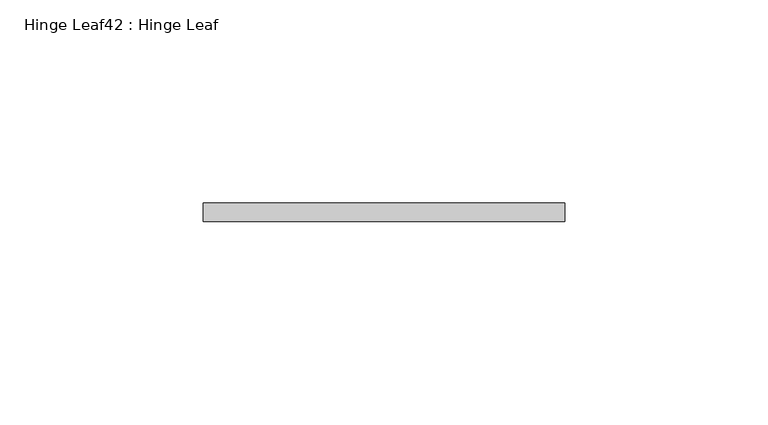
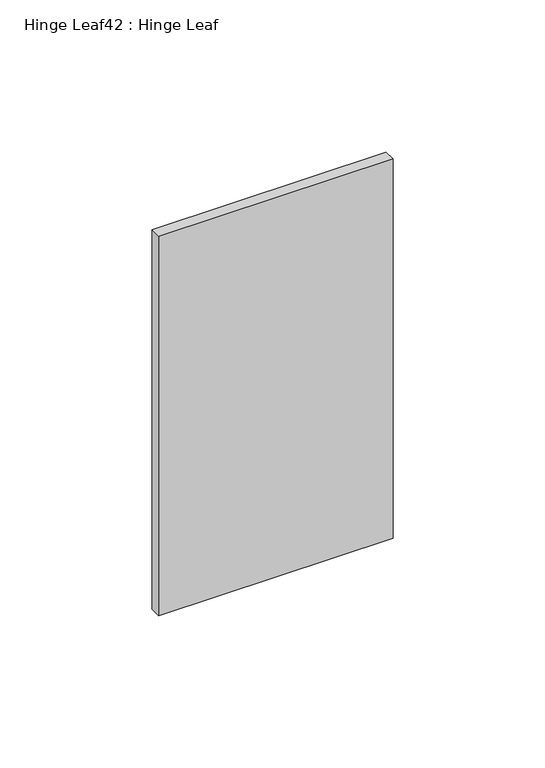
"""IFC4 building model written with IfcOpenShell, lengths in millimetres: proxy geometry, Hinge Leaf42 : Hinge Leaf."""

from ifc_helpers import new_model, si_unit, frame, origin, place, context, project, spatial, polyline, outline, extrude, source, transform, mapped, element, save


def hinge_leaf42_hinge_leaf_9b6187f5(model_context):
    return source(origin(), model_context, "Body", "SweptSolid", [
        extrude(outline(polyline([(587327.7934739, -534104.7943841), (587416.6934739, -534104.7943841), (587416.6934739, -534109.3663841), (587327.7934739, -534109.3663841), (587327.7934739, -534104.7943841)])), frame((0.0, 0.0, 1123.95), z_axis=(0.0, 0.0, 1.0), x_axis=(1.0, 0.0, 0.0)), (0.0, 0.0, 1.0), 152.4),
    ])


if __name__ == "__main__":
    model = new_model("IFC4")
    model_context = context("Model", 3, world=origin())
    ifc_project = project(units=[si_unit("LENGTHUNIT", "METRE", prefix="MILLI")], contexts=[model_context])
    site = spatial("IfcSite", under=ifc_project)
    building = spatial("IfcBuilding", under=site)
    placement = place(None, origin())
    hinge_leaf42_hinge_leaf_shape = hinge_leaf42_hinge_leaf_9b6187f5(model_context)
    element("IfcBuildingElementProxy", 1, Name="Hinge Leaf42 : Hinge Leaf", ObjectType="Hinge Leaf42 : Hinge Leaf", at=placement, inside=building, context=model_context, shape_type="MappedRepresentation", body=[
        mapped(hinge_leaf42_hinge_leaf_shape, transform((0.0, 0.0, 0.0), x_axis=(1.0, 0.0, 0.0), y_axis=(0.0, 1.0, 0.0), z_axis=(0.0, 0.0, 1.0))),
    ])
    save(model, "model.ifc")

# Revit data of these elements
# Element 1 (IfcBuildingElementProxy, "Hinge Leaf42 : Hinge Leaf")
#   Materials on its faces: "6\"X6\" WELD-ON STL BUTT HINGE"
# Materials
#   "6\"X6\" WELD-ON STL BUTT HINGE": class "Metal", colour RGB 189 187 185, transparency 0, Description = "Carbon steel", Cost = 0
